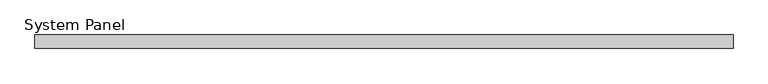
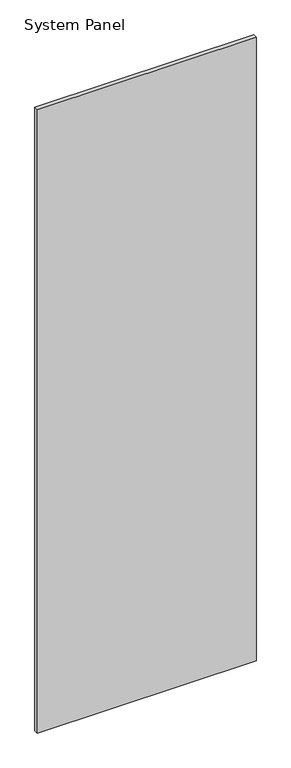
"""IFC4 building model written with IfcOpenShell, lengths in millimetres: plate geometry, System Panel : WWm-Glass-20mm-10mmOffset."""

from ifc_helpers import new_model, si_unit, origin, origin_with_axes, place, context, project, spatial, polyline, outline, extrude, source, transform, mapped, element, save


def system_panel_4c4673d4(model_context):
    return source(origin(), model_context, "Body", "SweptSolid", [
        extrude(outline(polyline([(522.7221833, 0.0), (-522.7221833, 0.0), (-522.7221833, 20.0), (522.7221833, 20.0), (522.7221833, 0.0)])), origin_with_axes(), (0.0, 0.0, 1.0), 3150.0),
    ])


if __name__ == "__main__":
    model = new_model("IFC4")
    model_context = context("Model", 3, world=origin())
    ifc_project = project(units=[si_unit("LENGTHUNIT", "METRE", prefix="MILLI")], contexts=[model_context])
    site = spatial("IfcSite", under=ifc_project)
    building = spatial("IfcBuilding", under=site)
    placement = place(None, origin())
    system_panel_shape = system_panel_4c4673d4(model_context)
    element("IfcPlate", 1, ObjectType="System Panel : WWm-Glass-20mm-10mmOffset", at=placement, inside=building, context=model_context, shape_type="MappedRepresentation", body=[
        mapped(system_panel_shape, transform((0.0, 0.0, 0.0), x_axis=(1.0, 0.0, 0.0), y_axis=(0.0, 1.0, 0.0), z_axis=(0.0, 0.0, 1.0))),
    ])
    save(model, "model.ifc")

# Revit data of these elements
# Type "System Panel : WWm-Glass-20mm-10mmOffset"
#   Finish = ""
# Element 1 (IfcPlate, "System Panel : WWm-Glass-20mm-10mmOffset")
#   Materials on its faces: "WW-EC-GL-Storefront"
# Materials
#   "WW-EC-GL-Storefront": class "Glass", colour RGB 236 240 239, transparency 0.85, Description = "Storefront Glass", Cost = 0
